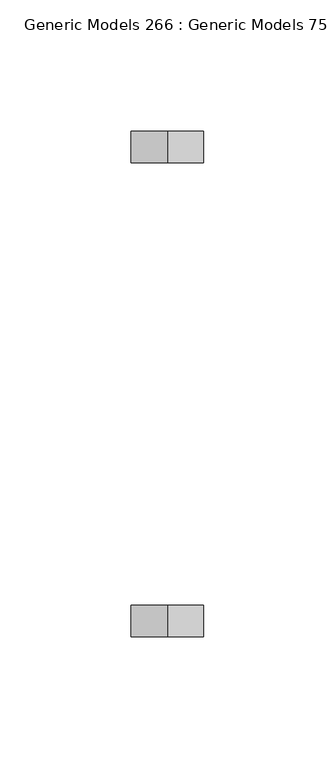
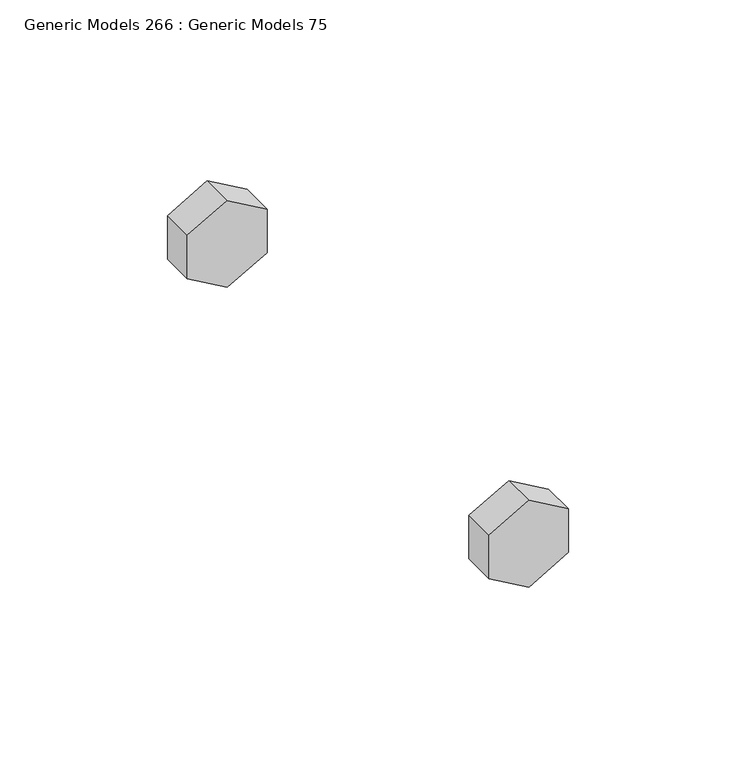
"""IFC4 building model written with IfcOpenShell, lengths in millimetres: proxy geometry, Generic Models 266 : Generic Models 75."""

from ifc_helpers import new_model, si_unit, frame, origin, place, context, project, spatial, polyline, outline, extrude, source, transform, mapped, element, save


def generic_models_266_generic_models_75_b6037518(model_context):
    return source(origin(), model_context, "Body", "SweptSolid", [
        extrude(outline(polyline([(268689.2902933, 31975.9942029), (268673.4537198, 31975.9942029), (268665.535433, 31989.7090778), (268673.4537198, 32003.4239528), (268689.2902933, 32003.4239528), (268697.20858, 31989.7090778), (268689.2902933, 31975.9942029)])), frame((0.0, 35373.9582942, 0.0), z_axis=(0.0, 1.0, 0.0), x_axis=(0.0, 0.0, 1.0)), (0.0, 0.0, 1.0), 11.90625),
        extrude(outline(polyline([(268689.2902933, 31975.9942029), (268673.4537198, 31975.9942029), (268665.535433, 31989.7090778), (268673.4537198, 32003.4239528), (268689.2902933, 32003.4239528), (268697.20858, 31989.7090778), (268689.2902933, 31975.9942029)])), frame((0.0, 35193.7770442, 0.0), z_axis=(0.0, 1.0, 0.0), x_axis=(0.0, 0.0, 1.0)), (0.0, 0.0, 1.0), 11.90625),
    ])


if __name__ == "__main__":
    model = new_model("IFC4")
    model_context = context("Model", 3, world=origin())
    ifc_project = project(units=[si_unit("LENGTHUNIT", "METRE", prefix="MILLI")], contexts=[model_context])
    site = spatial("IfcSite", under=ifc_project)
    building = spatial("IfcBuilding", under=site)
    placement = place(None, origin())
    generic_models_266_generic_models_75_shape = generic_models_266_generic_models_75_b6037518(model_context)
    element("IfcBuildingElementProxy", 1, Name="Generic Models 266 : Generic Models 75", ObjectType="Generic Models 266 : Generic Models 75", at=placement, inside=building, context=model_context, shape_type="MappedRepresentation", body=[
        mapped(generic_models_266_generic_models_75_shape, transform((0.0, 0.0, 0.0), x_axis=(1.0, 0.0, 0.0), y_axis=(0.0, 1.0, 0.0), z_axis=(0.0, 0.0, 1.0))),
    ])
    save(model, "model.ifc")

# Revit data of these elements
# Element 1 (IfcBuildingElementProxy, "Generic Models 266 : Generic Models 75")
#   Materials on its faces: "3/4\" GALV. THRU BOLTS"
# Materials
#   "3/4\" GALV. THRU BOLTS": class "Generic", colour RGB 105 69 171, transparency 0, Cost = 0
